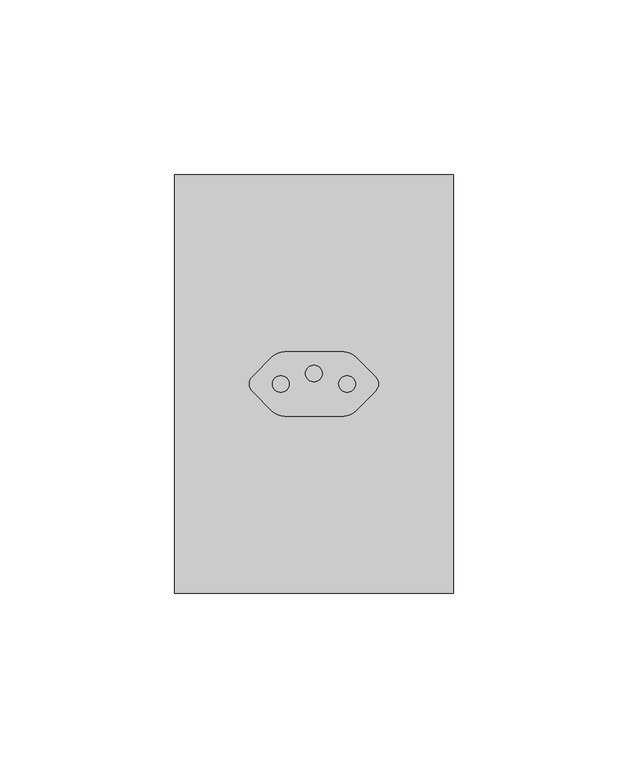
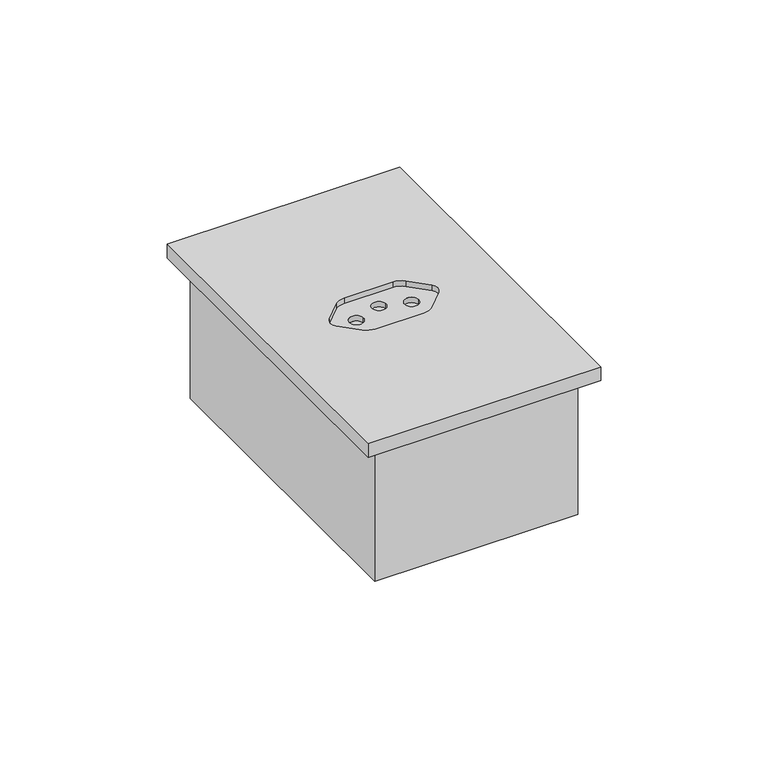
"""IFC4 building model written with IfcOpenShell, lengths in millimetres: proxy geometry, CAIXA VERTICE V7 : Tomada 20A 1s."""

from ifc_helpers import new_model, si_unit, frame, origin, place, context, project, spatial, polyline, circle_curve, faceted_brep, source, transform, mapped, element, save
from ifc_brep_helpers import plane_surface, revolved_surface, advanced_brep


def electrical_fixtures_cf860c52(model_context):
    return source(origin(), model_context, "Body", "SolidModel", [
        faceted_brep([(33.0, -53.0, -48.0), (33.0, 53.0, -48.0), (-33.0, 53.0, -48.0), (-33.0, -53.0, -48.0), (35.0, 55.0, -50.0), (35.0, -55.0, -50.0), (-35.0, -55.0, -50.0), (-35.0, 55.0, -50.0), (-35.0, 55.0, 0.0), (35.0, 55.0, 0.0), (-35.0, -55.0, 0.0), (35.0, -55.0, 0.0), (33.0, 53.0, 0.0), (33.0, -53.0, 0.0), (-33.0, -53.0, 0.0), (-33.0, 53.0, 0.0)], [[[0, 1, 2, 3]], [[4, 5, 6, 7]], [[4, 7, 8, 9]], [[8, 7, 6, 10]], [[10, 6, 5, 11]], [[11, 5, 4, 9]], [[9, 8, 10, 11], [12, 13, 14, 15]], [[13, 12, 1, 0]], [[14, 13, 0, 3]], [[15, 14, 3, 2]], [[12, 15, 2, 1]]]),
        advanced_brep(
        [(40.0, 60.0, 5.0), (-40.0, 60.0, 5.0), (-40.0, -60.0, 5.0), (40.0, -60.0, 5.0), (8.4215729, -9.25, 5.0), (-8.4215729, -9.25, 5.0), (-11.9571068, -7.7855339, 5.0), (-17.6213203, -2.1213203, 5.0), (-17.6213203, 2.1213203, 5.0), (-11.9571068, 7.7855339, 5.0), (-8.4215729, 9.25, 5.0), (8.4215729, 9.25, 5.0), (11.9571068, 7.7855339, 5.0), (17.6213203, 2.1213203, 5.0), (17.6213203, -2.1213203, 5.0), (11.9571068, -7.7855339, 5.0), (-40.0, 60.0, 0.0), (40.0, 60.0, 0.0), (40.0, -60.0, 0.0), (-40.0, -60.0, 0.0), (8.4215729, -9.25, 3.0), (11.9571068, -7.7855339, 3.0), (17.6213203, -2.1213203, 3.0), (17.6213203, 2.1213203, 3.0), (11.9571068, 7.7855339, 3.0), (8.4215729, 9.25, 3.0), (-8.4215729, 9.25, 3.0), (-11.9571068, 7.7855339, 3.0), (-17.6213203, 2.1213203, 3.0), (-17.6213203, -2.1213203, 3.0), (-11.9571068, -7.7855339, 3.0), (-8.4215729, -9.25, 3.0), (-7.1, 0.0, 3.0), (-11.9, 0.0, 3.0), (11.9, 0.0, 3.0), (7.1, 0.0, 3.0), (2.4, 3.0, 3.0), (-2.4, 3.0, 3.0), (-11.9, 0.0, 1.0), (-7.1, 0.0, 1.0), (7.1, 0.0, 1.0), (11.9, 0.0, 1.0), (-2.4, 3.0, 1.0), (2.4, 3.0, 1.0)],
        [
            (0, 1),
            (1, 2),
            (2, 3),
            (3, 0),
            (4, 5),
            (5, 6, circle_curve(frame((-8.4215729, -4.25, 5.0), z_axis=(0.0, 0.0, -1.0), x_axis=(-1.0, 0.0, 0.0)), 5.0)),
            (6, 7),
            (7, 8, circle_curve(frame((-15.5, 0.0, 5.0), z_axis=(0.0, 0.0, -1.0), x_axis=(-1.0, 0.0, 0.0)), 3.0)),
            (8, 9),
            (9, 10, circle_curve(frame((-8.4215729, 4.25, 5.0), z_axis=(0.0, 0.0, -1.0), x_axis=(-1.0, 0.0, 0.0)), 5.0)),
            (10, 11),
            (11, 12, circle_curve(frame((8.4215729, 4.25, 5.0), z_axis=(0.0, 0.0, -1.0), x_axis=(-1.0, 0.0, 0.0)), 5.0)),
            (12, 13),
            (13, 14, circle_curve(frame((15.5, 0.0, 5.0), z_axis=(0.0, 0.0, -1.0), x_axis=(-1.0, 0.0, 0.0)), 3.0)),
            (14, 15),
            (15, 4, circle_curve(frame((8.4215729, -4.25, 5.0), z_axis=(0.0, 0.0, -1.0), x_axis=(-1.0, 0.0, 0.0)), 5.0)),
            (16, 17),
            (17, 18),
            (18, 19),
            (19, 16),
            (0, 17),
            (16, 1),
            (19, 2),
            (18, 3),
            (20, 21, circle_curve(frame((8.4215729, -4.25, 3.0), z_axis=(0.0, 0.0, 1.0), x_axis=(-1.0, 0.0, 0.0)), 5.0)),
            (21, 22),
            (22, 23, circle_curve(frame((15.5, 0.0, 3.0), z_axis=(0.0, 0.0, 1.0), x_axis=(-1.0, 0.0, 0.0)), 3.0)),
            (23, 24),
            (24, 25, circle_curve(frame((8.4215729, 4.25, 3.0), z_axis=(0.0, 0.0, 1.0), x_axis=(-1.0, 0.0, 0.0)), 5.0)),
            (25, 26),
            (26, 27, circle_curve(frame((-8.4215729, 4.25, 3.0), z_axis=(0.0, 0.0, 1.0), x_axis=(-1.0, 0.0, 0.0)), 5.0)),
            (27, 28),
            (28, 29, circle_curve(frame((-15.5, 0.0, 3.0), z_axis=(0.0, 0.0, 1.0), x_axis=(-1.0, 0.0, 0.0)), 3.0)),
            (29, 30),
            (30, 31, circle_curve(frame((-8.4215729, -4.25, 3.0), z_axis=(0.0, 0.0, 1.0), x_axis=(-1.0, 0.0, 0.0)), 5.0)),
            (31, 20),
            (32, 33, circle_curve(frame((-9.5, 0.0, 3.0), z_axis=(0.0, 0.0, -1.0), x_axis=(1.0, 2.301812013077709e-12, 0.0)), 2.4)),
            (33, 32, circle_curve(frame((-9.5, 0.0, 3.0), z_axis=(0.0, 0.0, -1.0), x_axis=(1.0, 2.301812013077709e-12, 0.0)), 2.4)),
            (34, 35, circle_curve(frame((9.5, 0.0, 3.0), z_axis=(0.0, 0.0, -1.0), x_axis=(1.0, 2.301812013077709e-12, 0.0)), 2.4)),
            (35, 34, circle_curve(frame((9.5, 0.0, 3.0), z_axis=(0.0, 0.0, -1.0), x_axis=(1.0, 2.301812013077709e-12, 0.0)), 2.4)),
            (36, 37, circle_curve(frame((0.0, 3.0, 3.0), z_axis=(0.0, 0.0, -1.0), x_axis=(1.0, 2.301812013077709e-12, 0.0)), 2.4)),
            (37, 36, circle_curve(frame((0.0, 3.0, 3.0), z_axis=(0.0, 0.0, -1.0), x_axis=(1.0, 2.301812013077709e-12, 0.0)), 2.4)),
            (31, 5),
            (4, 20),
            (30, 6),
            (29, 7),
            (28, 8),
            (27, 9),
            (26, 10),
            (25, 11),
            (24, 12),
            (23, 13),
            (22, 14),
            (21, 15),
            (38, 39, circle_curve(frame((-9.5, 0.0, 1.0), z_axis=(0.0, 0.0, 1.0), x_axis=(1.0, 2.301812013077709e-12, 0.0)), 2.4)),
            (39, 38, circle_curve(frame((-9.5, 0.0, 1.0), z_axis=(0.0, 0.0, 1.0), x_axis=(1.0, 2.301812013077709e-12, 0.0)), 2.4)),
            (40, 41, circle_curve(frame((9.5, 0.0, 1.0), z_axis=(0.0, 0.0, 1.0), x_axis=(1.0, 2.301812013077709e-12, 0.0)), 2.4)),
            (41, 40, circle_curve(frame((9.5, 0.0, 1.0), z_axis=(0.0, 0.0, 1.0), x_axis=(1.0, 2.301812013077709e-12, 0.0)), 2.4)),
            (42, 43, circle_curve(frame((0.0, 3.0, 1.0), z_axis=(0.0, 0.0, 1.0), x_axis=(1.0, 2.301812013077709e-12, 0.0)), 2.4)),
            (43, 42, circle_curve(frame((0.0, 3.0, 1.0), z_axis=(0.0, 0.0, 1.0), x_axis=(1.0, 2.301812013077709e-12, 0.0)), 2.4)),
            (32, 39),
            (38, 33),
            (34, 41),
            (40, 35),
            (36, 43),
            (42, 37),
        ],
        [
            plane_surface(frame((-60.0, 60.0, 5.0), z_axis=(0.0, 0.0, 1.0), x_axis=(-1.0, 0.0, 0.0))),
            plane_surface(frame((-60.0, 60.0, 0.0), z_axis=(0.0, 0.0, -1.0), x_axis=(1.0, 0.0, 0.0))),
            plane_surface(frame((40.0, 60.0, 5.0), z_axis=(0.0, 1.0, 0.0), x_axis=(0.0, 0.0, -1.0))),
            plane_surface(frame((-40.0, 60.0, 5.0), z_axis=(-1.0, 0.0, 0.0), x_axis=(0.0, 0.0, -1.0))),
            plane_surface(frame((-40.0, -60.0, 5.0), z_axis=(0.0, -1.0, 0.0), x_axis=(0.0, 0.0, -1.0))),
            plane_surface(frame((40.0, -60.0, 5.0), z_axis=(1.0, 0.0, 0.0), x_axis=(0.0, 0.0, -1.0))),
            plane_surface(frame((3.4215729, -4.25, 3.0), z_axis=(0.0, 0.0, 1.0), x_axis=(0.0, 1.0, 0.0))),
            plane_surface(frame((-8.4215729, -9.25, 5.0), z_axis=(0.0, 1.0, 0.0), x_axis=(0.0, 0.0, -1.0))),
            revolved_surface(polyline([(-13.4215729, -4.25, 5.0), (-13.4215729, -4.25, 3.0)]), (-8.4215729, -4.25, 3.0), (0.0, 0.0, 1.0)),
            plane_surface(frame((-17.6213203, -2.1213203, 5.0), z_axis=(0.7071067811865045, 0.7071067811865905, 0.0), x_axis=(0.0, 0.0, -1.0))),
            revolved_surface(polyline([(-18.5, 0.0, 5.0), (-18.5, 0.0, 3.0)]), (-15.5, 0.0, 3.0), (0.0, 0.0, 1.0)),
            plane_surface(frame((-11.9571068, 7.7855339, 5.0), z_axis=(0.7071067811865515, -0.7071067811865437, 0.0), x_axis=(0.0, 0.0, -1.0))),
            revolved_surface(polyline([(-13.4215729, 4.25, 5.0), (-13.4215729, 4.25, 3.0)]), (-8.4215729, 4.25, 3.0), (0.0, 0.0, 1.0)),
            plane_surface(frame((8.4215729, 9.25, 5.0), z_axis=(0.0, -1.0, 0.0), x_axis=(0.0, 0.0, -1.0))),
            revolved_surface(polyline([(3.4215728999999993, 4.25, 5.0), (3.4215728999999993, 4.25, 3.0)]), (8.4215729, 4.25, 3.0), (0.0, 0.0, 1.0)),
            plane_surface(frame((17.6213203, 2.1213203, 5.0), z_axis=(-0.7071067811865307, -0.7071067811865643, 0.0), x_axis=(0.0, 0.0, -1.0))),
            revolved_surface(polyline([(12.5, 0.0, 5.0), (12.5, 0.0, 3.0)]), (15.5, 0.0, 3.0), (0.0, 0.0, 1.0)),
            plane_surface(frame((11.9571068, -7.7855339, 5.0), z_axis=(-0.7071067811865893, 0.7071067811865058, 0.0), x_axis=(0.0, 0.0, -1.0))),
            revolved_surface(polyline([(3.4215728999999993, -4.25, 5.0), (3.4215728999999993, -4.25, 3.0)]), (8.4215729, -4.25, 3.0), (0.0, 0.0, 1.0)),
            plane_surface(frame((-7.1, 0.0, 1.0), z_axis=(0.0, 0.0, 1.0), x_axis=(2.301812013077709e-12, -1.0, 0.0))),
            revolved_surface(polyline([(-7.1, 5.524348831386502e-12, 3.0), (-7.1, 5.524348831386502e-12, 1.0)]), (-9.5, 0.0, 1.0), (0.0, 0.0, 1.0)),
            revolved_surface(polyline([(11.9, 5.524348831386502e-12, 3.0), (11.9, 5.524348831386502e-12, 1.0)]), (9.5, 0.0, 5.0), (0.0, 0.0, 1.0)),
            revolved_surface(polyline([(2.4, 3.0000000000055245, 3.0), (2.4, 3.0000000000055245, 1.0)]), (0.0, 3.0, 5.0), (0.0, 0.0, 1.0)),
        ],
        [
            (0, [[1, 2, 3, 4], [5, 6, 7, 8, 9, 10, 11, 12, 13, 14, 15, 16]]),
            (1, [[17, 18, 19, 20]]),
            (2, [[-1, 21, -17, 22]]),
            (3, [[-2, -22, -20, 23]]),
            (4, [[-3, -23, -19, 24]]),
            (5, [[-4, -24, -18, -21]]),
            (6, [[25, 26, 27, 28, 29, 30, 31, 32, 33, 34, 35, 36], [37, 38], [39, 40], [41, 42]]),
            (7, [[-36, 43, -5, 44]]),
            (8, [[-35, 45, -6, -43]]),
            (9, [[-34, 46, -7, -45]]),
            (10, [[-33, 47, -8, -46]]),
            (11, [[-32, 48, -9, -47]]),
            (12, [[-31, 49, -10, -48]]),
            (13, [[-30, 50, -11, -49]]),
            (14, [[-29, 51, -12, -50]]),
            (15, [[-28, 52, -13, -51]]),
            (16, [[-27, 53, -14, -52]]),
            (17, [[-26, 54, -15, -53]]),
            (18, [[-25, -44, -16, -54]]),
            (19, [[55, 56]]),
            (19, [[57, 58]]),
            (19, [[59, 60]]),
            (20, [[-37, 61, -55, 62]]),
            (20, [[-38, -62, -56, -61]]),
            (21, [[-39, 63, -57, 64]]),
            (21, [[-40, -64, -58, -63]]),
            (22, [[-41, 65, -59, 66]]),
            (22, [[-42, -66, -60, -65]]),
        ],
    ),
    ])


if __name__ == "__main__":
    model = new_model("IFC4")
    model_context = context("Model", 3, world=origin())
    ifc_project = project(units=[si_unit("LENGTHUNIT", "METRE", prefix="MILLI")], contexts=[model_context])
    site = spatial("IfcSite", under=ifc_project)
    building = spatial("IfcBuilding", under=site)
    placement = place(None, origin())
    electrical_fixtures_shape = electrical_fixtures_cf860c52(model_context)
    element("IfcBuildingElementProxy", 1, Name="CAIXA VERTICE V7 : Tomada 20A 1s", ObjectType="CAIXA VERTICE V7 : Tomada 20A 1s", at=placement, inside=building, context=model_context, shape_type="MappedRepresentation", body=[
        mapped(electrical_fixtures_shape, transform((0.0, 0.0, 0.0), x_axis=(1.0, 0.0, 0.0), y_axis=(0.0, 1.0, 0.0), z_axis=(0.0, 0.0, 1.0))),
    ])
    save(model, "model.ifc")

# Revit data of these elements
# Type "CAIXA VERTICE V7 : Tomada 20A 1s"
#   URL = "www.facebook.com/verticetreinamentos"
#   SEÇÃO [instance default] = ""
#   Rotação [instance default] = 0.00°
#   LARGURA DA TAMPA = 0.08 m
#   BORDA = 0.01 m
#   ALTURA DE INSTALAÇÃO [instance default] = 1.10 m
#   Distância Anotação [instance default] = 0.0015 m
#   ALTURA DA TAMPA = 0.12 m
#   Vertical [instance default] = yes
#   VER SEÇÃO [instance default] = no
#   SHADE ESQ [instance default] = no
#   SHADE DIR [instance default] = yes
#   HORIZONTAL [instance default] = no
#   ANDAR COM A LEGENDA [instance default] = 0
#   Material Tampa [instance default] = Plástico, branco opaco
#   Caixa = element 1798517
#   Anotação = element 1798531
#   Default Elevation = 0
# Element 1 (IfcBuildingElementProxy, "CAIXA VERTICE V7 : Tomada 20A 1s")
#   ALTURA DE INSTALAÇÃO = 0.00 m
#   SHADE DIR = no
#   Materials on its faces: "Plástico, branco opaco"
# Materials
#   "Plástico, branco opaco": class "Plástico", colour RGB 120 120 120, transparency 0, Description = "Plastic, generic, opaque white", Cost = 0
